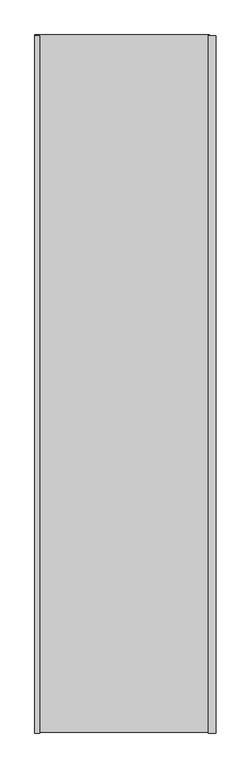
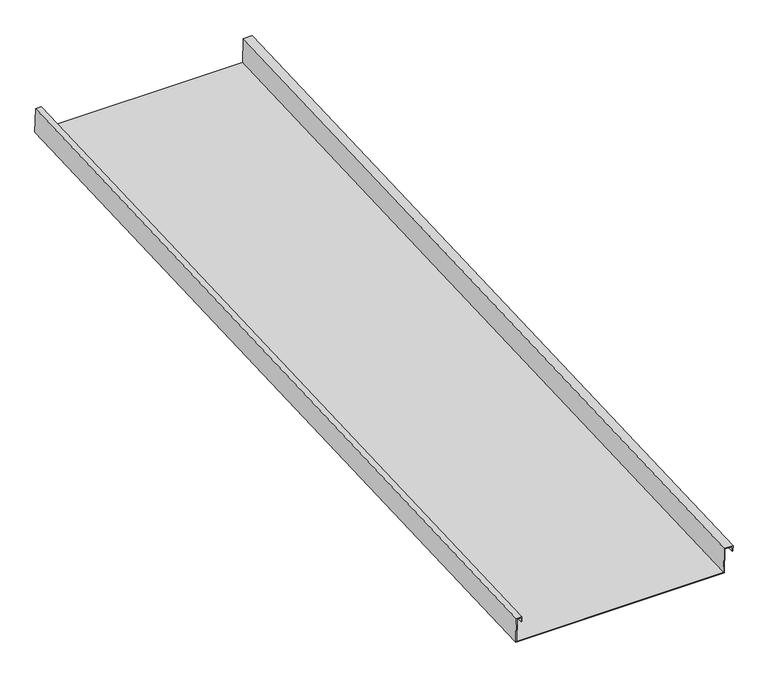
"""IFC4 building model written with IfcOpenShell, lengths in millimetres: proxy geometry, Generic Models 2:Generic Models 2:310765:Generic Models 2:310765 : Generic Models 2:Generic Models 2:310765:21 : Generic Models 2:Generic Models 2:310765:Generic Models 2:310765 : Generic Models 2:Generic Models 2:310765:300385."""

from ifc_helpers import new_model, si_unit, origin, place, context, project, spatial, faceted_brep, source, transform, mapped, element, save


def generic_models_c28749cd(model_context):
    return source(origin(), model_context, "Body", "Brep", [
        faceted_brep([(579578.4218144, -580678.4204475, 3889.8483266), (579578.4218144, -580680.5352791, 3940.6042867), (579592.7093144, -580680.5352791, 3940.6042867), (579592.7093144, -580680.1387482, 3931.0875442), (579594.2968144, -580680.1387482, 3931.0875442), (579594.2968144, -580680.6013676, 3942.1904105), (579576.8343144, -580680.6013676, 3942.1904105), (579576.8343144, -580678.4865359, 3891.4344503), (579173.6093144, -580678.4865359, 3891.4344503), (579173.6093144, -580680.4031021, 3937.4320392), (579181.5468144, -580680.4031021, 3937.4320392), (579181.5468144, -580680.0726597, 3929.5014204), (579183.1343144, -580680.0726597, 3929.5014204), (579183.1343144, -580680.4691906, 3939.018163), (579172.0218144, -580680.4691906, 3939.018163), (579172.0218144, -580678.4204475, 3889.8483266), (579592.7093144, -579057.8507862, 3998.6828759), (579592.7093144, -579058.2473171, 4008.1996185), (579591.201064, -579058.2473171, 4008.1996185), (579578.4218144, -579058.2473171, 4008.1996185), (579578.4218144, -579056.1324855, 3957.4436583), (579576.913564, -579056.1324855, 3957.4436583), (579354.663564, -579056.1324855, 3957.4436583), (579172.0218144, -579056.1324855, 3957.4436583), (579172.0218144, -579058.1812286, 4006.6134947), (579183.1343144, -579058.1812286, 4006.6134947), (579183.1343144, -579057.7846977, 3997.0967522), (579181.5468144, -579057.7846977, 3997.0967522), (579181.5468144, -579058.1151401, 4005.027371), (579173.6093144, -579058.1151401, 4005.027371), (579173.6093144, -579056.1985739, 3959.0297821), (579354.663564, -579056.1985739, 3959.0297821), (579356.251064, -579056.1985739, 3959.0297821), (579575.326064, -579056.1985739, 3959.0297821), (579576.8343144, -579056.1985739, 3959.0297821), (579576.8343144, -579058.2473171, 4008.1996185), (579576.8343144, -579058.3134056, 4009.7857422), (579592.788564, -579058.3134056, 4009.7857422), (579594.2968144, -579058.3134056, 4009.7857422), (579594.2968144, -579057.8507862, 3998.6828759)], [[[0, 1, 2, 3, 4, 5, 6, 7, 8, 9, 10, 11, 12, 13, 14, 15]], [[16, 17, 18, 19, 20, 21, 22, 23, 24, 25, 26, 27, 28, 29, 30, 31, 32, 33, 34, 35, 36, 37, 38, 39]], [[2, 1, 19, 18, 17]], [[17, 16, 3, 2]], [[16, 39, 4, 3]], [[39, 38, 5, 4]], [[6, 5, 38, 37, 36]], [[7, 6, 36, 35, 34]], [[8, 7, 34, 33, 32, 31, 30]], [[30, 29, 9, 8]], [[29, 28, 10, 9]], [[28, 27, 11, 10]], [[27, 26, 12, 11]], [[26, 25, 13, 12]], [[25, 24, 14, 13]], [[24, 23, 15, 14]], [[0, 15, 23, 22, 21, 20]], [[20, 19, 1, 0]]]),
    ])


if __name__ == "__main__":
    model = new_model("IFC4")
    model_context = context("Model", 3, world=origin())
    ifc_project = project(units=[si_unit("LENGTHUNIT", "METRE", prefix="MILLI")], contexts=[model_context])
    site = spatial("IfcSite", under=ifc_project)
    building = spatial("IfcBuilding", under=site)
    placement = place(None, origin())
    generic_models_shape = generic_models_c28749cd(model_context)
    element("IfcBuildingElementProxy", 1, Name="Generic Models 2:Generic Models 2:310765:Generic Models 2:310765 : Generic Models 2:Generic Models 2:310765:21 : Generic Models 2:Generic Models 2:310765:Generic Models 2:310765 : Generic Models 2:Generic Models 2:310765:300385", ObjectType="Generic Models 2:Generic Models 2:310765:Generic Models 2:310765 : Generic Models 2:Generic Models 2:310765:21 : Generic Models 2:Generic Models 2:310765:Generic Models 2:310765 : Generic Models 2:Generic Models 2:310765:300385", at=placement, inside=building, context=model_context, shape_type="MappedRepresentation", body=[
        mapped(generic_models_shape, transform((0.0, 0.0, 0.0), x_axis=(1.0, 0.0, 0.0), y_axis=(0.0, 1.0, 0.0), z_axis=(0.0, 0.0, 1.0))),
    ])
    save(model, "model.ifc")

# Revit data of these elements
# Type "Generic Models 2:Generic Models 2:310765:Generic Models 2:310765 : Generic Models 2:Generic Models 2:310765:21 : Generic Models 2:Generic Models 2:310765:Generic Models 2:310765 : Generic Models 2:Generic Models 2:310765:300385"
#   NameOverride = "Generic Models 2:Generic Models 2:310765:Generic Models 2:310765 : Generic Models 2:Generic Models 2:310765:300385"
#   ObjectTypeOverride = "Generic Models 2:310765 : Generic Models 2:Generic Models 2:310765"
#   Reference = "Generic Models 2"
#   Tag = "300385"
# Element 1 (IfcBuildingElementProxy, "Generic Models 2:Generic Models 2:310765:Generic Models 2:310765 : Generic Models 2:Generic Models 2:310765:21 : Generic Models 2:Generic Models 2:310765:Generic Models 2:310765 : Generic Models 2:Generic Models 2:310765:300385")
#   Materials on its faces: "STRUCTURAL STANDING SEAM SHEET METAL ROOFING - BATTENLOK - COLOR T.B.D."
# Materials
#   "STRUCTURAL STANDING SEAM SHEET METAL ROOFING - BATTENLOK - COLOR T.B.D.": class "Generic", colour RGB 120 120 120, transparency 0, Cost = 0
